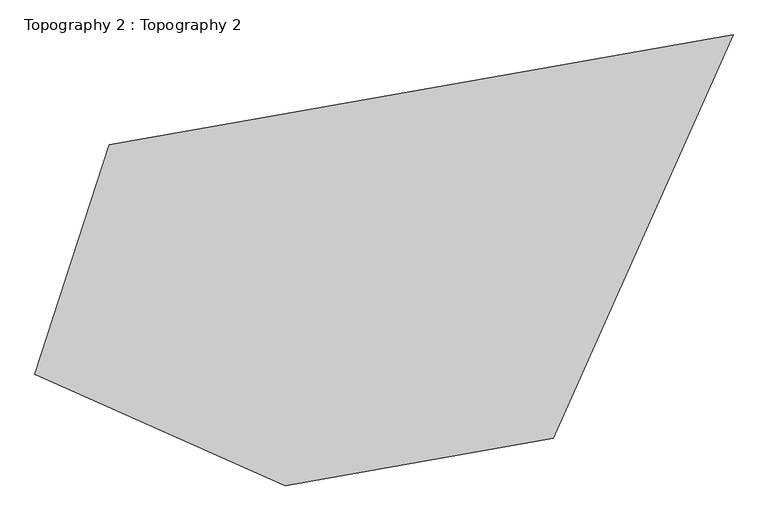
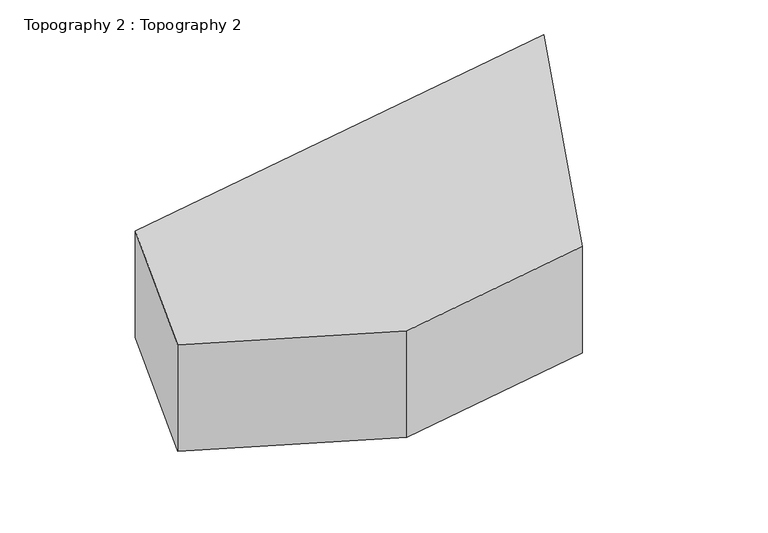
"""IFC4 building model written with IfcOpenShell, lengths in millimetres: proxy geometry, Topography 2 : Topography 2."""

from ifc_helpers import new_model, si_unit, frame, origin, place, context, project, spatial, polyline, outline, extrude, source, transform, mapped, element, save


def topography_2_topography_2_0c5f490f(model_context):
    return source(origin(), model_context, "Body", "SweptSolid", [
        extrude(outline(polyline([(149937.6623725, 96245.9914351), (180817.6408186, 101690.9647988), (171924.0736635, 81715.6859173), (158639.5949547, 79373.2738963), (146247.9969154, 84890.3688002), (149937.6623725, 96245.9914351)])), frame((0.0, 0.0, -10770.0), z_axis=(0.0, 0.0, 1.0), x_axis=(1.0, 0.0, 0.0)), (0.0, 0.0, 1.0), 7660.6217624),
    ])


if __name__ == "__main__":
    model = new_model("IFC4")
    model_context = context("Model", 3, world=origin())
    ifc_project = project(units=[si_unit("LENGTHUNIT", "METRE", prefix="MILLI")], contexts=[model_context])
    site = spatial("IfcSite", under=ifc_project)
    building = spatial("IfcBuilding", under=site)
    placement = place(None, origin())
    topography_2_topography_2_shape = topography_2_topography_2_0c5f490f(model_context)
    element("IfcBuildingElementProxy", 1, Name="Topography 2 : Topography 2", ObjectType="Topography 2 : Topography 2", at=placement, inside=building, context=model_context, shape_type="MappedRepresentation", body=[
        mapped(topography_2_topography_2_shape, transform((0.0, 0.0, 0.0), x_axis=(1.0, 0.0, 0.0), y_axis=(0.0, 1.0, 0.0), z_axis=(0.0, 0.0, 1.0))),
    ])
    save(model, "model.ifc")

# Revit data of these elements
# Element 1 (IfcBuildingElementProxy, "Topography 2 : Topography 2")
#   Materials on its faces: "Earth"
# Materials
#   "Earth": class "Generic", colour RGB 97 75 62, transparency 0, Description = "Soil", Cost = 0
